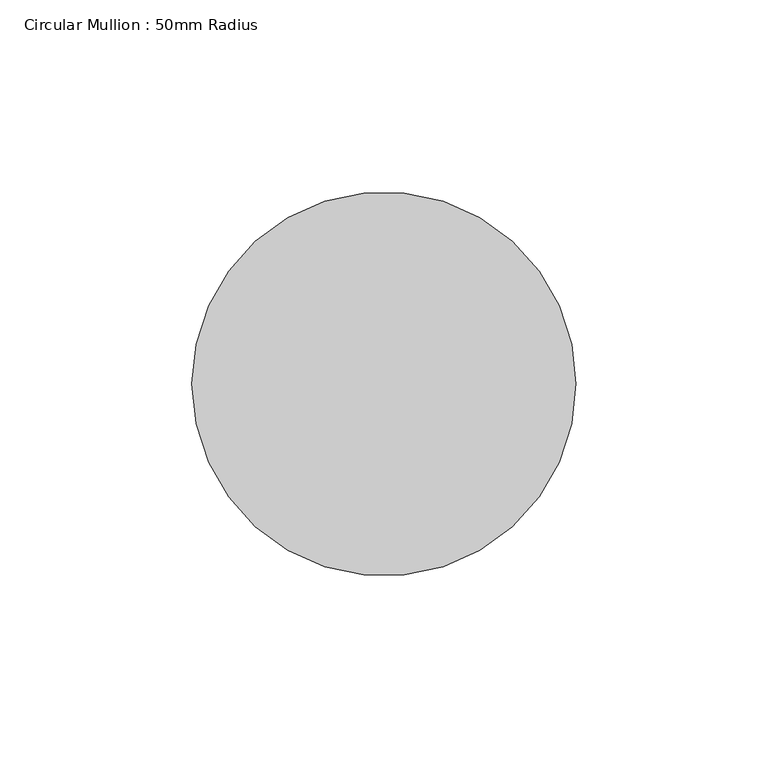
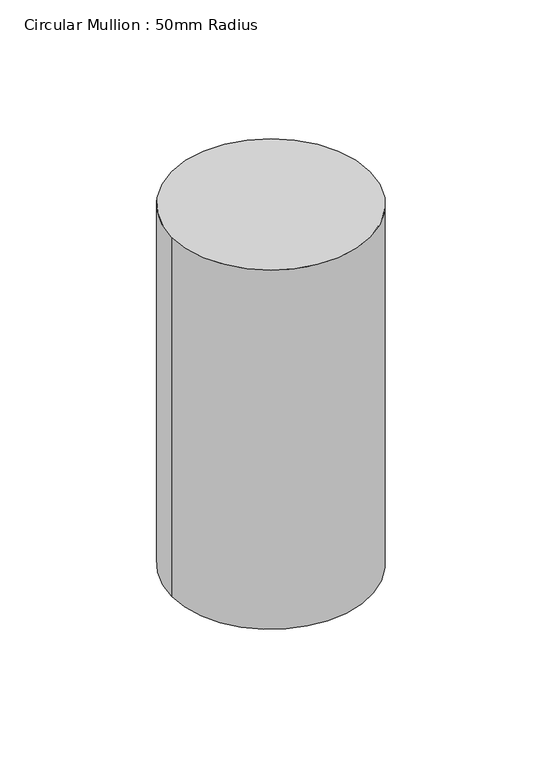
"""IFC4 building model written with IfcOpenShell, lengths in millimetres: member geometry, Circular Mullion : 50mm Radius."""

from ifc_helpers import new_model, si_unit, point, frame, origin, origin_2d, place, context, project, spatial, circle_curve, trimmed, segment, composite_curve, outline, extrude, source, transform, mapped, element, save


def circular_mullion_50mm_radius_e2a65007(model_context):
    return source(origin(), model_context, "Body", "SweptSolid", [
        extrude(outline(composite_curve([segment(trimmed(circle_curve(origin_2d(), 50.0), [point((50.0, 0.0))], [point((-50.0, 0.0))], False, "CARTESIAN"), True, "CONTINUOUS"), segment(trimmed(circle_curve(origin_2d(), 50.0), [point((-50.0, 0.0))], [point((50.0, 0.0))], False, "CARTESIAN"), True, "CONTINUOUS")], self_intersect=False)), frame((0.0, 0.0, -191.3655043), z_axis=(0.0, 0.0, 1.0), x_axis=(1.0, 0.0, 0.0)), (0.0, 0.0, 1.0), 191.3655043),
    ])


if __name__ == "__main__":
    model = new_model("IFC4")
    model_context = context("Model", 3, world=origin())
    ifc_project = project(units=[si_unit("LENGTHUNIT", "METRE", prefix="MILLI")], contexts=[model_context])
    site = spatial("IfcSite", under=ifc_project)
    building = spatial("IfcBuilding", under=site)
    placement = place(None, origin())
    circular_mullion_50mm_radius_shape = circular_mullion_50mm_radius_e2a65007(model_context)
    element("IfcMember", 1, ObjectType="Circular Mullion : 50mm Radius", at=placement, inside=building, context=model_context, shape_type="MappedRepresentation", body=[
        mapped(circular_mullion_50mm_radius_shape, transform((0.0, 0.0, 0.0), x_axis=(1.0, 0.0, 0.0), y_axis=(0.0, 1.0, 0.0), z_axis=(0.0, 0.0, 1.0))),
    ])
    save(model, "model.ifc")

# Revit data of these elements
# Type "Circular Mullion : 50mm Radius"
#   built-in parameter 1007350 = 0.164042 (stored number, unit not read)
# Element 1 (IfcMember, "Circular Mullion : 50mm Radius")
#   Materials on its faces: "Aluminium"
# Materials
#   "Aluminium": class "Metal", colour RGB 247 247 247, transparency 0, Description = "Aluminium 6061", Cost = 0
